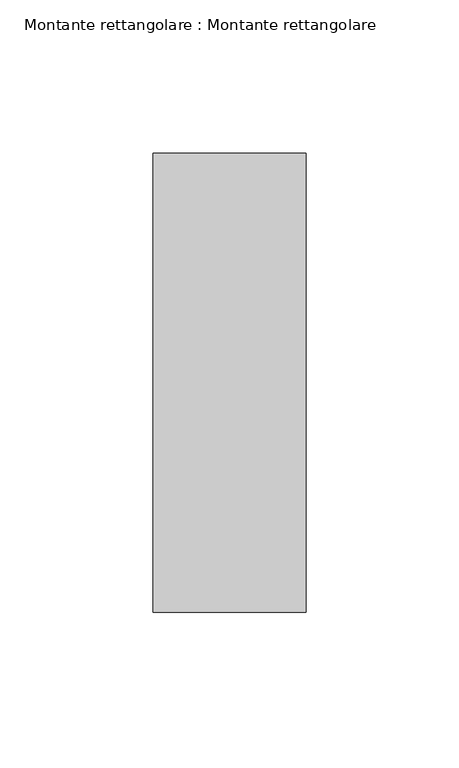
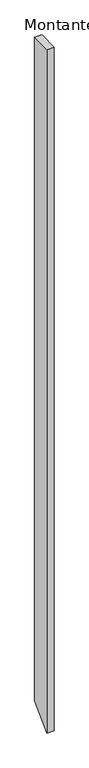
"""IFC4 building model written with IfcOpenShell, lengths in millimetres: member geometry, Montante rettangolare : Montante rettangolare."""

from ifc_helpers import new_model, si_unit, frame, origin, place, context, project, spatial, polyline, outline, extrude, source, transform, mapped, element, save


def montante_rettangolare_montante_rettangolare_9078f481(model_context):
    return source(origin(), model_context, "Body", "SweptSolid", [
        extrude(outline(polyline([(-75.0, 0.0), (75.0, 0.0), (75.0, -4930.0), (-75.0, -5080.0), (-75.0, 0.0)])), frame((-50.0, 0.0, 0.0), z_axis=(1.0, 0.0, 0.0), x_axis=(0.0, 1.0, 0.0)), (0.0, 0.0, 1.0), 50.0),
    ])


if __name__ == "__main__":
    model = new_model("IFC4")
    model_context = context("Model", 3, world=origin())
    ifc_project = project(units=[si_unit("LENGTHUNIT", "METRE", prefix="MILLI")], contexts=[model_context])
    site = spatial("IfcSite", under=ifc_project)
    building = spatial("IfcBuilding", under=site)
    placement = place(None, origin())
    montante_rettangolare_montante_rettangolare_shape = montante_rettangolare_montante_rettangolare_9078f481(model_context)
    element("IfcMember", 1, ObjectType="Montante rettangolare : Montante rettangolare", at=placement, inside=building, context=model_context, shape_type="MappedRepresentation", body=[
        mapped(montante_rettangolare_montante_rettangolare_shape, transform((0.0, 0.0, 0.0), x_axis=(1.0, 0.0, 0.0), y_axis=(0.0, 1.0, 0.0), z_axis=(0.0, 0.0, 1.0))),
    ])
    save(model, "model.ifc")

# Revit data of these elements
# Type "Montante rettangolare : Montante rettangolare"
#   built-in parameter 1007304 = 0.492126 (stored number, unit not read)
#   built-in parameter 1007301 = 0.082021 (stored number, unit not read)
#   built-in parameter 1007300 = 0.082021 (stored number, unit not read)
# Element 1 (IfcMember, "Montante rettangolare : Montante rettangolare")
#   Materials on its faces: "Acciaio"
# Materials
#   "Acciaio": class "Metallo", colour RGB 247 247 247, transparency 0, Description = "Acciaio, finitura zigrinata", Cost = 0
